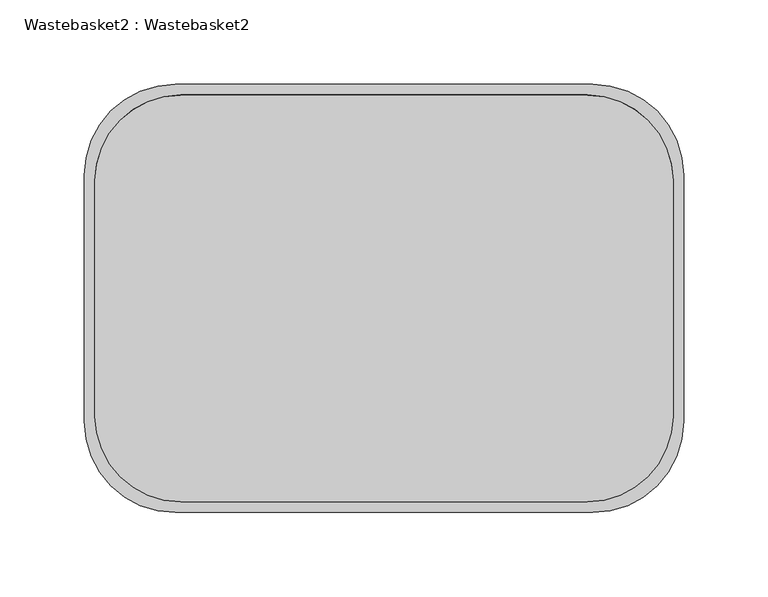
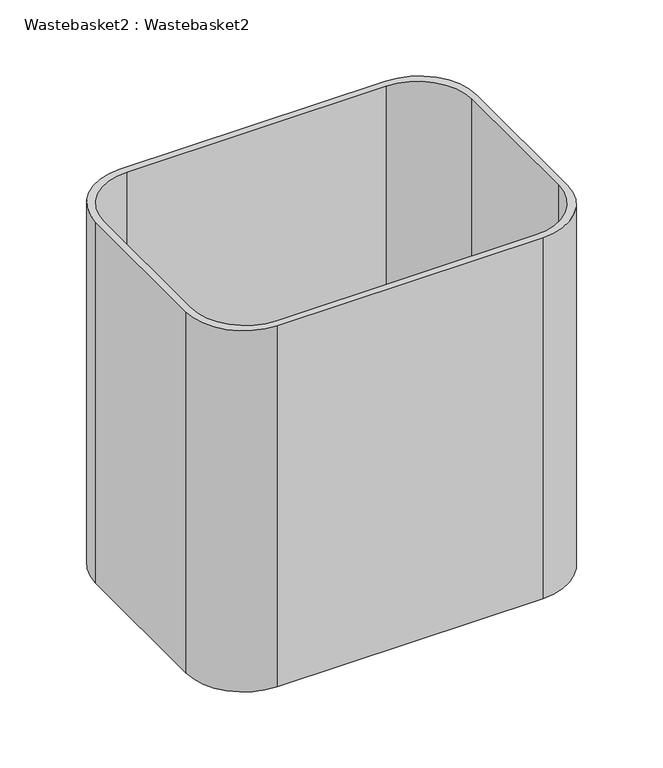
"""IFC4 building model written with IfcOpenShell, lengths in millimetres: furniture geometry, Wastebasket2 : Wastebasket2."""

import ifcopenshell
import ifcopenshell.guid

model = None  # the IFC model being written
_history = None  # IfcOwnerHistory: only IFC2X3 demands one
_inside = {}  # id of a spatial element -> (the spatial element, [elements in it])
_under = {}  # id of a project, library or spatial element -> (it, [spatial elements below it])
_declared = {}  # id of a project -> (the project, [libraries it declares])
_typed = {}  # id of a type object -> (the type object, [elements of that type])
_made_of = {}  # id of a material, layer set ... -> (it, [elements and type objects made of it])


def new_model(schema):
    """Start an empty IFC model of exactly this schema.

    Asked for "IFC4X3", IfcOpenShell would pick the latest addendum, in which some entities
    have other attributes; the version numbers below select the first issue.
    IFC2X3 requires an IfcOwnerHistory on every rooted entity: one is made here for all.
    """
    global model, _history
    if schema == "IFC4X3":
        model = ifcopenshell.file(schema_version=(4, 3, 0, 0))
    else:
        model = ifcopenshell.file(schema=schema)
    _inside.clear()
    _under.clear()
    _declared.clear()
    _typed.clear()
    _made_of.clear()
    _history = None
    if model.schema == "IFC2X3":
        org = make("IfcOrganization", Name="unknown")
        user = make(
            "IfcPersonAndOrganization",
            ThePerson=make("IfcPerson", FamilyName="unknown"),
            TheOrganization=org,
        )
        app = make(
            "IfcApplication",
            ApplicationDeveloper=org,
            Version="unknown",
            ApplicationFullName="unknown",
            ApplicationIdentifier="unknown",
        )
        _history = make(
            "IfcOwnerHistory",
            OwningUser=user,
            OwningApplication=app,
            ChangeAction="ADDED",
            CreationDate=0,
        )
    return model


def make(cls, **values):
    """One entity of the class cls with the attributes given. An attribute that is None is left unset."""
    return model.create_entity(
        cls, **{name: value for name, value in values.items() if value is not None}
    )


def rooted(cls, **values):
    """An entity with a GlobalId (a new one), such as an element, a storey or a relation."""
    return make(cls, GlobalId=ifcopenshell.guid.new(), OwnerHistory=_history, **values)


def si_unit(unit_type, name, prefix=None):
    """IfcSIUnit, for example si_unit("LENGTHUNIT", "METRE", prefix="MILLI")."""
    return make("IfcSIUnit", UnitType=unit_type, Prefix=prefix, Name=name)


def assignment(units):
    """IfcUnitAssignment: the units of a project."""
    return None if units is None else make("IfcUnitAssignment", Units=units)


def point(xyz):
    """IfcCartesianPoint."""
    return None if xyz is None else make("IfcCartesianPoint", Coordinates=xyz)


def direction(xyz):
    """IfcDirection."""
    return None if xyz is None else make("IfcDirection", DirectionRatios=xyz)


def frame(location, z_axis=None, x_axis=None):
    """IfcAxis2Placement3D, a coordinate frame: its origin and axes. An axis left out is left unset."""
    return make(
        "IfcAxis2Placement3D",
        Location=point(location),
        Axis=direction(z_axis),
        RefDirection=direction(x_axis),
    )


def origin():
    """The frame at (0, 0, 0) with its axes left unset."""
    return frame((0.0, 0.0, 0.0))


def place(relative_to, where):
    """IfcLocalPlacement: puts the frame where relative to a parent placement (None: the world)."""
    return make(
        "IfcLocalPlacement", PlacementRelTo=relative_to, RelativePlacement=where
    )


def context(
    kind, dimensions, precision=None, world=None, true_north=None, identifier=None
):
    """IfcGeometricRepresentationContext, for example the 3D "Model" context."""
    return make(
        "IfcGeometricRepresentationContext",
        ContextIdentifier=identifier,
        ContextType=kind,
        CoordinateSpaceDimension=dimensions,
        Precision=precision,
        WorldCoordinateSystem=world,
        TrueNorth=true_north,
    )


def project(units=None, contexts=None):
    """IfcProject with its units and contexts."""
    return rooted(
        "IfcProject",
        Name="project",
        RepresentationContexts=contexts,
        UnitsInContext=assignment(units),
    )


def spatial(cls, under=None, at=None, **own):
    """A site, building, storey or space (cls), placed at a placement, below another one or the project."""
    s = rooted(cls, ObjectPlacement=at, **own)
    if under is not None:
        _under.setdefault(under.id(), (under, []))[1].append(s)
    return s


def polyline(points):
    """IfcPolyline through the points."""
    return make("IfcPolyline", Points=[point(p) for p in points])


def circle_curve(where, radius):
    """IfcCircle in the frame where."""
    return make("IfcCircle", Position=where, Radius=radius)


def shape(context_of_items, identifier, shape_type, items):
    """IfcShapeRepresentation: the items that make up one representation, for example the "Body"."""
    return make(
        "IfcShapeRepresentation",
        ContextOfItems=context_of_items,
        RepresentationIdentifier=identifier,
        RepresentationType=shape_type,
        Items=items,
    )


def source(mapping_origin, context_of_items, identifier, shape_type, items):
    """IfcRepresentationMap: a shape defined once, which mapped items show again and again."""
    return make(
        "IfcRepresentationMap",
        MappingOrigin=mapping_origin,
        MappedRepresentation=shape(context_of_items, identifier, shape_type, items),
    )


def transform(
    local_origin,
    x_axis=None,
    y_axis=None,
    z_axis=None,
    scale=None,
    scale2=None,
    scale3=None,
    uniform=True,
):
    """IfcCartesianTransformationOperator3D, or its non-uniform kind. x_axis, y_axis, z_axis: its Axis1, 2, 3."""
    if uniform:
        return make(
            "IfcCartesianTransformationOperator3D",
            Axis1=direction(x_axis),
            Axis2=direction(y_axis),
            LocalOrigin=point(local_origin),
            Scale=scale,
            Axis3=direction(z_axis),
        )
    return make(
        "IfcCartesianTransformationOperator3DnonUniform",
        Axis1=direction(x_axis),
        Axis2=direction(y_axis),
        LocalOrigin=point(local_origin),
        Scale=scale,
        Axis3=direction(z_axis),
        Scale2=scale2,
        Scale3=scale3,
    )


def mapped(mapping_source, mapping_target):
    """IfcMappedItem: shows the shape of a source again, moved by a transform."""
    return make(
        "IfcMappedItem", MappingSource=mapping_source, MappingTarget=mapping_target
    )


def made_of(thing, what):
    """Note that an element or type object is made of a material, layer set ...; save() writes the relation."""
    if what is not None:
        _made_of.setdefault(what.id(), (what, []))[1].append(thing)
    return thing


def element(
    cls,
    number,
    at=None,
    inside=None,
    cuts=None,
    type_object=None,
    material=None,
    context=None,
    identifier="Body",
    shape_type=None,
    held_by="IfcProductDefinitionShape",
    body=None,
    shapes=None,
    **own,
):
    """One element of the class cls, such as IfcWall. Its Tag is "e" and its number.

    at: its placement. inside: the storey or other place that contains it. cuts: it is an
    opening in that element (IfcRelVoidsElement). A single representation is given by context,
    identifier, shape_type and body (its items); several are given by shapes. held_by: the class
    of the entity that holds the representations. save() writes the other relations.
    """
    e = rooted(cls, Tag="e%d" % number, ObjectPlacement=at, **own)
    if body is not None:
        shapes = [shape(context, identifier, shape_type, body)]
    if shapes is not None:
        e.Representation = make(held_by, Representations=shapes)
    if inside is not None:
        _inside.setdefault(inside.id(), (inside, []))[1].append(e)
    if cuts is not None:
        rooted(
            "IfcRelVoidsElement", RelatingBuildingElement=cuts, RelatedOpeningElement=e
        )
    if type_object is not None:
        _typed.setdefault(type_object.id(), (type_object, []))[1].append(e)
    return made_of(e, material)


def aggregate(whole, parts):
    """IfcRelAggregates: a whole, such as a stair, and the parts it consists of."""
    return rooted("IfcRelAggregates", RelatingObject=whole, RelatedObjects=parts)


def save(model, path):
    """Write the relations noted so far, then the file.

    IfcRelAggregates (storeys below a building ...), IfcRelContainedInSpatialStructure (elements
    in a storey), IfcRelDefinesByType, IfcRelAssociatesMaterial and IfcRelDeclares: one each for
    every whole, place, type object, material and project.
    """
    for whole, parts in _under.values():
        aggregate(whole, parts)
    for where, things in _inside.values():
        rooted(
            "IfcRelContainedInSpatialStructure",
            RelatedElements=things,
            RelatingStructure=where,
        )
    for kind, things in _typed.values():
        rooted("IfcRelDefinesByType", RelatedObjects=things, RelatingType=kind)
    for what, things in _made_of.values():
        rooted("IfcRelAssociatesMaterial", RelatedObjects=things, RelatingMaterial=what)
    for by, libraries in _declared.values():
        rooted("IfcRelDeclares", RelatingContext=by, RelatedDefinitions=libraries)
    model.write(path)


def plane_surface(at):
    """IfcPlane: the flat surface through the origin of the frame at, square to its z axis."""
    return make("IfcPlane", Position=at)


def cylinder_surface(at, radius):
    """IfcCylindricalSurface: all points at the distance radius from the z axis of the frame at."""
    return make("IfcCylindricalSurface", Position=at, Radius=radius)


def revolved_surface(curve, axis_point, axis_direction):
    """IfcSurfaceOfRevolution: the curve turned about the line through axis_point along axis_direction."""
    return make(
        "IfcSurfaceOfRevolution",
        SweptCurve=make("IfcArbitraryOpenProfileDef", ProfileType="CURVE", Curve=curve),
        AxisPosition=make("IfcAxis1Placement", Location=point(axis_point), Axis=direction(axis_direction)),
    )


def advanced_brep(points, edges, surfaces, faces):
    """IfcAdvancedBrep: a solid bounded by faces that lie on surfaces and meet in shared edges.

    An edge is (start, end): straight between two places in points (the first is 0);
    or (start, end, curve); or (start, end, curve, False) where it runs against its curve.
    A face is (place in surfaces, loops), or (place, loops, False) where it looks against
    its surface's normal. A loop lists edges by number (the first is 1), with a minus sign
    where the edge is run from its end to its start. The first loop is the outer one.
    """
    corners = [point(p) for p in points]
    vertices = [make("IfcVertexPoint", VertexGeometry=c) for c in corners]
    made = []
    for start, end, *more in edges:
        made.append(
            make(
                "IfcEdgeCurve",
                EdgeStart=vertices[start],
                EdgeEnd=vertices[end],
                EdgeGeometry=more[0] if more else make("IfcPolyline", Points=[corners[start], corners[end]]),
                SameSense=more[1] if len(more) > 1 else True,
            )
        )
    hull = []
    for where, loops, *sense in faces:
        bounds = []
        for j, loop in enumerate(loops):
            ring = [make("IfcOrientedEdge", EdgeElement=made[abs(k) - 1], Orientation=k > 0) for k in loop]
            bounds.append(
                make(
                    "IfcFaceOuterBound" if j == 0 else "IfcFaceBound",
                    Bound=make("IfcEdgeLoop", EdgeList=ring),
                    Orientation=True,
                )
            )
        hull.append(make("IfcAdvancedFace", Bounds=bounds, FaceSurface=surfaces[where], SameSense=sense[0] if sense else True))
    return make("IfcAdvancedBrep", Outer=make("IfcClosedShell", CfsFaces=hull))


def wastebasket2_wastebasket2_e1224e57(model_context):
    return source(origin(), model_context, "Body", "AdvancedBrep", [
        advanced_brep(
        [(178.3203994, 170.9615385, 355.6), (-69.3296006, 170.9615385, 355.6), (-123.3046006, 116.9865385, 355.6), (-123.3046006, -29.0634615, 355.6), (-69.3296006, -83.0384615, 355.6), (178.3203994, -83.0384615, 355.6), (232.2953994, -29.0634615, 355.6), (232.2953994, 116.9865385, 355.6), (-66.1546006, 164.6115385, 355.6), (175.1453994, 164.6115385, 355.6), (225.9453994, 113.8115385, 355.6), (225.9453994, -25.8884615, 355.6), (175.1453994, -76.6884615, 355.6), (-66.1546006, -76.6884615, 355.6), (-116.9546006, -25.8884615, 355.6), (-116.9546006, 113.8115385, 355.6), (178.3203994, 170.9615385, 0.0), (232.2953994, 116.9865385, 0.0), (232.2953994, -29.0634615, 0.0), (178.3203994, -83.0384615, 0.0), (-69.3296006, -83.0384615, 0.0), (-123.3046006, -29.0634615, 0.0), (-123.3046006, 116.9865385, 0.0), (-69.3296006, 170.9615385, 0.0), (175.1453994, 164.6115385, 12.7), (-66.1546006, 164.6115385, 12.7), (-116.9546006, 113.8115385, 12.7), (-116.9546006, -25.8884615, 12.7), (-66.1546006, -76.6884615, 12.7), (175.1453994, -76.6884615, 12.7), (225.9453994, -25.8884615, 12.7), (225.9453994, 113.8115385, 12.7)],
        [
            (0, 1),
            (1, 2, circle_curve(frame((-69.3296006, 116.9865385, 355.6), z_axis=(0.0, 0.0, 1.0), x_axis=(1.0, 0.0, 0.0)), 53.975)),
            (2, 3),
            (3, 4, circle_curve(frame((-69.3296006, -29.0634615, 355.6), z_axis=(0.0, 0.0, 1.0), x_axis=(1.0, 0.0, 0.0)), 53.975)),
            (4, 5),
            (5, 6, circle_curve(frame((178.3203994, -29.0634615, 355.6), z_axis=(0.0, 0.0, 1.0), x_axis=(1.0, 0.0, 0.0)), 53.975)),
            (6, 7),
            (7, 0, circle_curve(frame((178.3203994, 116.9865385, 355.6), z_axis=(0.0, 0.0, 1.0), x_axis=(1.0, 0.0, 0.0)), 53.975)),
            (8, 9),
            (9, 10, circle_curve(frame((175.1453994, 113.8115385, 355.6), z_axis=(0.0, 0.0, -1.0), x_axis=(1.0, 0.0, 0.0)), 50.8)),
            (10, 11),
            (11, 12, circle_curve(frame((175.1453994, -25.8884615, 355.6), z_axis=(0.0, 0.0, -1.0), x_axis=(1.0, 0.0, 0.0)), 50.8)),
            (12, 13),
            (13, 14, circle_curve(frame((-66.1546006, -25.8884615, 355.6), z_axis=(0.0, 0.0, -1.0), x_axis=(1.0, 0.0, 0.0)), 50.8)),
            (14, 15),
            (15, 8, circle_curve(frame((-66.1546006, 113.8115385, 355.6), z_axis=(0.0, 0.0, -1.0), x_axis=(1.0, 0.0, 0.0)), 50.8)),
            (16, 17, circle_curve(frame((178.3203994, 116.9865385, 0.0), z_axis=(0.0, 0.0, -1.0), x_axis=(1.0, 0.0, 0.0)), 53.975)),
            (17, 18),
            (18, 19, circle_curve(frame((178.3203994, -29.0634615, 0.0), z_axis=(0.0, 0.0, -1.0), x_axis=(1.0, 0.0, 0.0)), 53.975)),
            (19, 20),
            (20, 21, circle_curve(frame((-69.3296006, -29.0634615, 0.0), z_axis=(0.0, 0.0, -1.0), x_axis=(1.0, 0.0, 0.0)), 53.975)),
            (21, 22),
            (22, 23, circle_curve(frame((-69.3296006, 116.9865385, 0.0), z_axis=(0.0, 0.0, -1.0), x_axis=(1.0, 0.0, 0.0)), 53.975)),
            (23, 16),
            (0, 16),
            (23, 1),
            (22, 2),
            (21, 3),
            (20, 4),
            (19, 5),
            (18, 6),
            (17, 7),
            (24, 25),
            (25, 26, circle_curve(frame((-66.1546006, 113.8115385, 12.7), z_axis=(0.0, 0.0, 1.0), x_axis=(1.0, 0.0, 0.0)), 50.8)),
            (26, 27),
            (27, 28, circle_curve(frame((-66.1546006, -25.8884615, 12.7), z_axis=(0.0, 0.0, 1.0), x_axis=(1.0, 0.0, 0.0)), 50.8)),
            (28, 29),
            (29, 30, circle_curve(frame((175.1453994, -25.8884615, 12.7), z_axis=(0.0, 0.0, 1.0), x_axis=(1.0, 0.0, 0.0)), 50.8)),
            (30, 31),
            (31, 24, circle_curve(frame((175.1453994, 113.8115385, 12.7), z_axis=(0.0, 0.0, 1.0), x_axis=(1.0, 0.0, 0.0)), 50.8)),
            (24, 9),
            (8, 25),
            (15, 26),
            (14, 27),
            (13, 28),
            (12, 29),
            (11, 30),
            (10, 31),
        ],
        [
            plane_surface(frame((-123.3046006, 170.9615385, 355.6), z_axis=(0.0, 0.0, 1.0), x_axis=(-1.0, 0.0, 0.0))),
            plane_surface(frame((-123.3046006, 170.9615385, 0.0), z_axis=(0.0, 0.0, -1.0), x_axis=(1.0, 0.0, 0.0))),
            plane_surface(frame((178.3203994, 170.9615385, 355.6), z_axis=(0.0, 1.0, 0.0), x_axis=(0.0, 0.0, -1.0))),
            cylinder_surface(frame((-69.3296006, 116.9865385, 0.0), z_axis=(0.0, 0.0, 1.0), x_axis=(1.0, 0.0, 0.0)), 53.975),
            plane_surface(frame((-123.3046006, 116.9865385, 355.6), z_axis=(-1.0, 0.0, 0.0), x_axis=(0.0, 0.0, -1.0))),
            cylinder_surface(frame((-69.3296006, -29.0634615, 0.0), z_axis=(0.0, 0.0, 1.0), x_axis=(1.0, 0.0, 0.0)), 53.975),
            plane_surface(frame((-69.3296006, -83.0384615, 355.6), z_axis=(0.0, -1.0, 0.0), x_axis=(0.0, 0.0, -1.0))),
            cylinder_surface(frame((178.3203994, -29.0634615, 0.0), z_axis=(0.0, 0.0, 1.0), x_axis=(1.0, 0.0, 0.0)), 53.975),
            plane_surface(frame((232.2953994, -29.0634615, 355.6), z_axis=(1.0, 0.0, 0.0), x_axis=(0.0, 0.0, -1.0))),
            cylinder_surface(frame((178.3203994, 116.9865385, 0.0), z_axis=(0.0, 0.0, 1.0), x_axis=(1.0, 0.0, 0.0)), 53.975),
            plane_surface(frame((-66.1546006, 164.6115385, 12.7), z_axis=(0.0, 0.0, 1.0), x_axis=(1.0, 0.0, 0.0))),
            plane_surface(frame((175.1453994, 164.6115385, 355.6), z_axis=(0.0, -1.0, 0.0), x_axis=(0.0, 0.0, -1.0))),
            revolved_surface(polyline([(-15.354600599999998, 113.8115385, 355.6), (-15.354600599999998, 113.8115385, 12.7)]), (-66.1546006, 113.8115385, 12.7), (0.0, 0.0, 1.0)),
            plane_surface(frame((-116.9546006, 113.8115385, 355.6), z_axis=(1.0, 0.0, 0.0), x_axis=(0.0, 0.0, -1.0))),
            revolved_surface(polyline([(-15.354600599999998, -25.8884615, 355.6), (-15.354600599999998, -25.8884615, 12.7)]), (-66.1546006, -25.8884615, 12.7), (0.0, 0.0, 1.0)),
            plane_surface(frame((-66.1546006, -76.6884615, 355.6), z_axis=(0.0, 1.0, 0.0), x_axis=(0.0, 0.0, -1.0))),
            revolved_surface(polyline([(225.94539939999999, -25.8884615, 355.6), (225.94539939999999, -25.8884615, 12.7)]), (175.1453994, -25.8884615, 12.7), (0.0, 0.0, 1.0)),
            plane_surface(frame((225.9453994, -25.8884615, 355.6), z_axis=(-1.0, 0.0, 0.0), x_axis=(0.0, 0.0, -1.0))),
            revolved_surface(polyline([(225.94539939999999, 113.8115385, 355.6), (225.94539939999999, 113.8115385, 12.7)]), (175.1453994, 113.8115385, 12.7), (0.0, 0.0, 1.0)),
        ],
        [
            (0, [[1, 2, 3, 4, 5, 6, 7, 8], [9, 10, 11, 12, 13, 14, 15, 16]]),
            (1, [[17, 18, 19, 20, 21, 22, 23, 24]]),
            (2, [[-1, 25, -24, 26]]),
            (3, [[-2, -26, -23, 27]]),
            (4, [[-3, -27, -22, 28]]),
            (5, [[-4, -28, -21, 29]]),
            (6, [[-5, -29, -20, 30]]),
            (7, [[-6, -30, -19, 31]]),
            (8, [[-7, -31, -18, 32]]),
            (9, [[-8, -32, -17, -25]]),
            (10, [[33, 34, 35, 36, 37, 38, 39, 40]]),
            (11, [[-33, 41, -9, 42]]),
            (12, [[-34, -42, -16, 43]]),
            (13, [[-35, -43, -15, 44]]),
            (14, [[-36, -44, -14, 45]]),
            (15, [[-37, -45, -13, 46]]),
            (16, [[-38, -46, -12, 47]]),
            (17, [[-39, -47, -11, 48]]),
            (18, [[-40, -48, -10, -41]]),
        ],
    ),
    ])


if __name__ == "__main__":
    model = new_model("IFC4")
    model_context = context("Model", 3, world=origin())
    ifc_project = project(units=[si_unit("LENGTHUNIT", "METRE", prefix="MILLI")], contexts=[model_context])
    site = spatial("IfcSite", under=ifc_project)
    building = spatial("IfcBuilding", under=site)
    placement = place(None, origin())
    wastebasket2_wastebasket2_shape = wastebasket2_wastebasket2_e1224e57(model_context)
    element("IfcFurniture", 1, ObjectType="Wastebasket2 : Wastebasket2", at=placement, inside=building, context=model_context, shape_type="MappedRepresentation", body=[
        mapped(wastebasket2_wastebasket2_shape, transform((0.0, 0.0, 0.0), x_axis=(1.0, 0.0, 0.0), y_axis=(0.0, 1.0, 0.0), z_axis=(0.0, 0.0, 1.0))),
    ])
    save(model, "model.ifc")

# Revit data of these elements
# Type "Wastebasket2 : Wastebasket2"
#   Default Elevation = 0
#   Assembly Code = ""
# Element 1 (IfcFurniture, "Wastebasket2 : Wastebasket2")
#   Materials on its faces: "Metal - Chrome"
# Materials
#   "Metal - Chrome": class "Unassigned", colour RGB 17 17 17, transparency 0
